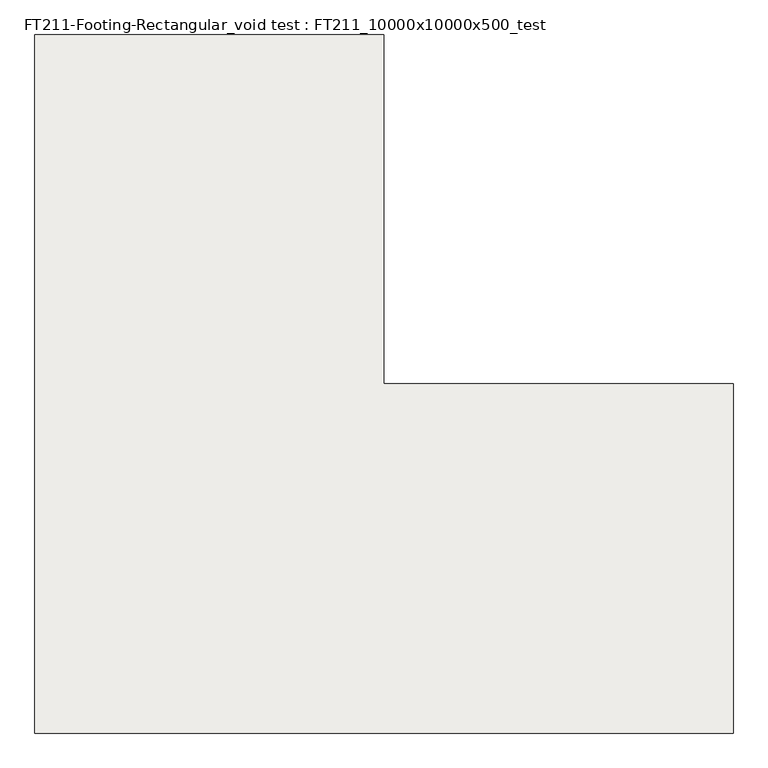
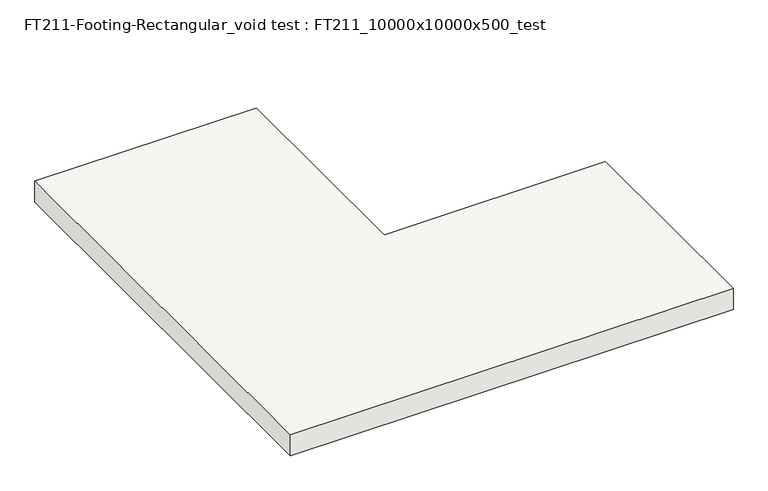
"""IFC4 building model written with IfcOpenShell, lengths in millimetres: slab geometry, FT211-Footing-Rectangular_void test : FT211_10000x10000x500_test."""

from ifc_helpers import new_model, si_unit, frame, origin, place, context, project, spatial, polyline, outline, extrude, source, transform, mapped, element, save


def ft211_footing_rectangular_void_test_ft211_10000x10000x500_68336e3b(model_context):
    return source(origin(), model_context, "Body", "SweptSolid", [
        extrude(outline(polyline([(5000.0, -5000.0), (-5000.0, -5000.0), (-5000.0, 5000.0), (0.0, 5000.0), (0.0, 0.0), (5000.0, 0.0), (5000.0, -5000.0)])), frame((0.0, 0.0, -500.0), z_axis=(0.0, 0.0, 1.0), x_axis=(1.0, 0.0, 0.0)), (0.0, 0.0, 1.0), 500.0),
    ])


if __name__ == "__main__":
    model = new_model("IFC4")
    model_context = context("Model", 3, world=origin())
    ifc_project = project(units=[si_unit("LENGTHUNIT", "METRE", prefix="MILLI")], contexts=[model_context])
    site = spatial("IfcSite", under=ifc_project)
    building = spatial("IfcBuilding", under=site)
    placement = place(None, origin())
    ft211_footing_rectangular_void_test_ft211_10000x10000x500_shape = ft211_footing_rectangular_void_test_ft211_10000x10000x500_68336e3b(model_context)
    element("IfcSlab", 1, ObjectType="FT211-Footing-Rectangular_void test : FT211_10000x10000x500_test", at=placement, inside=building, context=model_context, shape_type="MappedRepresentation", body=[
        mapped(ft211_footing_rectangular_void_test_ft211_10000x10000x500_shape, transform((0.0, 0.0, 0.0), x_axis=(1.0, 0.0, 0.0), y_axis=(0.0, 1.0, 0.0), z_axis=(0.0, 0.0, 1.0))),
    ])
    save(model, "model.ifc")

# Revit data of these elements
# Type "FT211-Footing-Rectangular_void test : FT211_10000x10000x500_test"
#   Top bar = "D25@300"
#   Description = "UG Shallow Foundation"
#   Bottom bar = "D20@300"
#   Width = 10000 mm
#   Length = 10000 mm
#   Foundation Thickness = 500 mm
#   Structural Material [instance default] = A03AC032-00007_Structural Concrete_Type1_25MPa-30Mpa
#   Assembly Code = ""
# Element 1 (IfcSlab, "FT211-Footing-Rectangular_void test : FT211_10000x10000x500_test")
#   Materials on its faces: "A03AC032-00007_Structural Concrete_Type1_25MPa-30Mpa"
# Materials
#   "A03AC032-00007_Structural Concrete_Type1_25MPa-30Mpa": class "Concrete", colour RGB 176 176 176, transparency 0, Keynote = "09910.A1", Description = "Reinf. Conc.", W00) Work Master Code = "A03AC032-00007", W01) Work Master_Lv1 = "Concrete Work", W02) Work Master_Lv2 = "Substructure Work", W03) Work Master_Spec.1 = "Structural Concrete", W04) Work Master_Spec.2 = "Cement Type-1", W05) Work Master_Spec.3 = "25MPa < F'c (Cylinder Strength) ≤ 30MPa", Cost = 0
